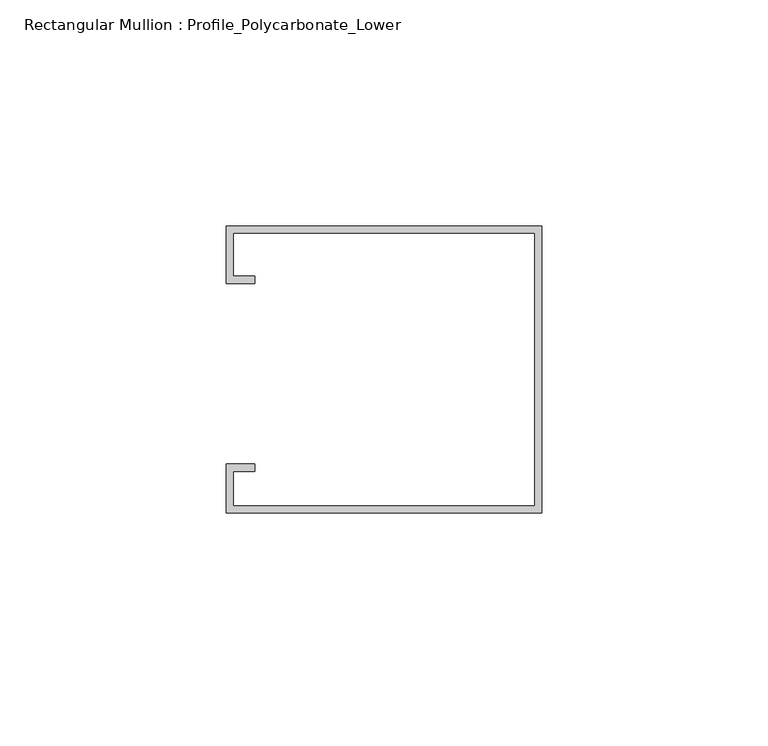
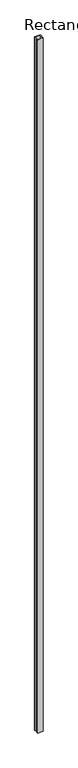
"""IFC4 building model written with IfcOpenShell, lengths in millimetres: member geometry, Rectangular Mullion : Profile_Polycarbonate_Lower."""

from ifc_helpers import new_model, si_unit, frame, origin, place, context, project, spatial, polyline, outline, extrude, source, transform, mapped, element, save


def rectangular_mullion_profile_polycarbonate_lower_ef4c2cf9(model_context):
    return source(origin(), model_context, "Body", "SweptSolid", [
        extrude(outline(polyline([(0.0, 32.7), (0.0, -30.8), (-69.85, -30.8), (-69.85, -20.0), (-63.5, -20.0), (-63.5, -21.5875), (-68.2625, -21.5875), (-68.2625, -29.2125), (-1.5875, -29.2125), (-1.5875, 31.1125), (-68.2625, 31.1125), (-68.2625, 21.5875), (-63.5, 21.5875), (-63.5, 20.0), (-69.85, 20.0), (-69.85, 32.7), (0.0, 32.7)])), frame((0.0, 0.0, -9101.1375), z_axis=(0.0, 0.0, 1.0), x_axis=(1.0, 0.0, 0.0)), (0.0, 0.0, 1.0), 9101.1375),
    ])


if __name__ == "__main__":
    model = new_model("IFC4")
    model_context = context("Model", 3, world=origin())
    ifc_project = project(units=[si_unit("LENGTHUNIT", "METRE", prefix="MILLI")], contexts=[model_context])
    site = spatial("IfcSite", under=ifc_project)
    building = spatial("IfcBuilding", under=site)
    placement = place(None, origin())
    rectangular_mullion_profile_polycarbonate_lower_shape = rectangular_mullion_profile_polycarbonate_lower_ef4c2cf9(model_context)
    element("IfcMember", 1, ObjectType="Rectangular Mullion : Profile_Polycarbonate_Lower", at=placement, inside=building, context=model_context, shape_type="MappedRepresentation", body=[
        mapped(rectangular_mullion_profile_polycarbonate_lower_shape, transform((0.0, 0.0, 0.0), x_axis=(1.0, 0.0, 0.0), y_axis=(0.0, 1.0, 0.0), z_axis=(0.0, 0.0, 1.0))),
    ])
    save(model, "model.ifc")

# Revit data of these elements
# Type "Rectangular Mullion : Profile_Polycarbonate_Lower"
#   built-in parameter 1007322 = 0.208333 (stored number, unit not read)
#   built-in parameter 1007321 = 0 (stored number, unit not read)
#   built-in parameter 1007320 = 0.00520833 (stored number, unit not read)
# Element 1 (IfcMember, "Rectangular Mullion : Profile_Polycarbonate_Lower")
#   Materials on its faces: "ALUMINUM PROFILE AT POLYCARBONATE PANEL"
# Materials
#   "ALUMINUM PROFILE AT POLYCARBONATE PANEL": class "Metal", colour RGB 244 244 244, transparency 0, Description = "Aluminum 6061", Cost = 0
